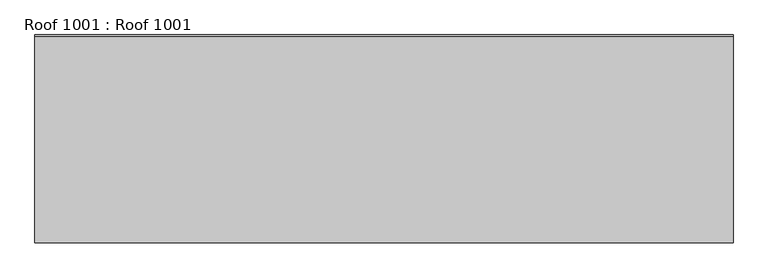
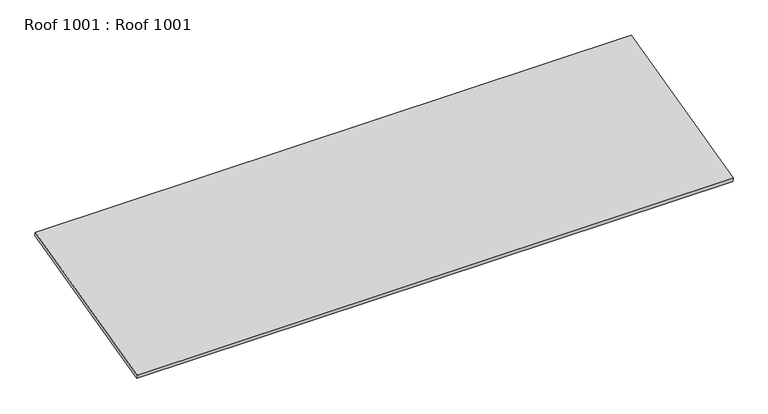
"""IFC4 building model written with IfcOpenShell, lengths in millimetres: proxy geometry, Roof 1001 : Roof 1001."""

from ifc_helpers import new_model, si_unit, frame, origin, place, context, project, spatial, polyline, outline, extrude, source, transform, mapped, element, save


def roof_1001_roof_1001_a34b083e(model_context):
    return source(origin(), model_context, "Body", "SweptSolid", [
        extrude(outline(polyline([(10172.9326802, 43745.1772707), (10169.629843, 43758.3886195), (10762.0851937, 43906.5005553), (10765.3875834, 43893.2909965), (10172.9326802, 43745.1772707)])), frame((3694.2883192, 0.0, 0.0), z_axis=(1.0, 0.0, 0.0), x_axis=(0.0, 1.0, 0.0)), (0.0, 0.0, 1.0), 2000.0),
    ])


if __name__ == "__main__":
    model = new_model("IFC4")
    model_context = context("Model", 3, world=origin())
    ifc_project = project(units=[si_unit("LENGTHUNIT", "METRE", prefix="MILLI")], contexts=[model_context])
    site = spatial("IfcSite", under=ifc_project)
    building = spatial("IfcBuilding", under=site)
    placement = place(None, origin())
    roof_1001_roof_1001_shape = roof_1001_roof_1001_a34b083e(model_context)
    element("IfcBuildingElementProxy", 1, Name="Roof 1001 : Roof 1001", ObjectType="Roof 1001 : Roof 1001", at=placement, inside=building, context=model_context, shape_type="MappedRepresentation", body=[
        mapped(roof_1001_roof_1001_shape, transform((0.0, 0.0, 0.0), x_axis=(1.0, 0.0, 0.0), y_axis=(0.0, 1.0, 0.0), z_axis=(0.0, 0.0, 1.0))),
    ])
    save(model, "model.ifc")

# Revit data of these elements
# Type "Roof 1001 : Roof 1001"
#   NameOverride = "Roof"
# Element 1 (IfcBuildingElementProxy, "Roof 1001 : Roof 1001")
#   Materials on its faces: "STANDING SEAM METAL ROOF"
# Materials
#   "STANDING SEAM METAL ROOF": class "Unassigned", colour RGB 128 128 128, transparency 0
